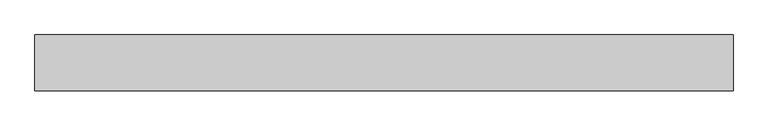
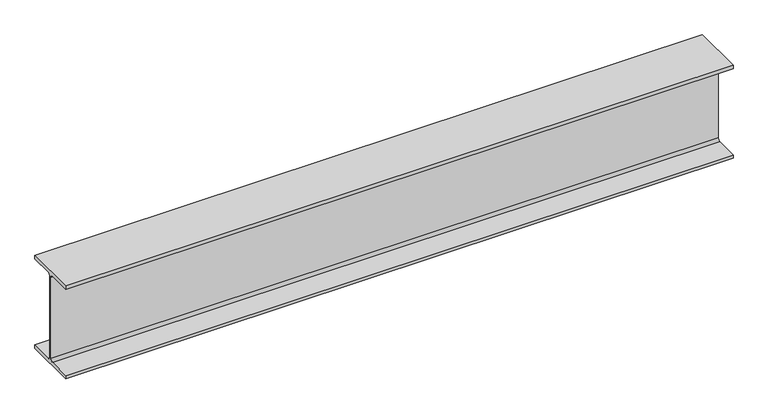
"""IFC4 building model written with IfcOpenShell, lengths in millimetres: beam geometry, Old_Steel Beam_H-KSD3502 : H_SB_ASB_H-194×150x6x9."""

from ifc_helpers import new_model, si_unit, point, frame, frame_2d, origin, place, context, project, spatial, polyline, circle_curve, trimmed, segment, composite_curve, outline, extrude, source, transform, mapped, element, save


def beam_5794e32c(model_context):
    return source(origin(), model_context, "Body", "SweptSolid", [
        extrude(outline(composite_curve([segment(polyline([(82.5, -141.5), (82.5, -151.7), (-82.5, -151.7), (-82.5, -141.5), (-11.9, -141.5)]), True, "CONTINUOUS"), segment(trimmed(circle_curve(frame_2d((-11.9, -132.6)), 8.9), [point((-11.9, -141.5))], [point((-3.0, -132.6))], True, "CARTESIAN"), True, "CONTINUOUS"), segment(polyline([(-3.0, -132.6), (-3.0, 132.6)]), True, "CONTINUOUS"), segment(trimmed(circle_curve(frame_2d((-11.9, 132.6)), 8.9), [point((-3.0, 132.6))], [point((-11.9, 141.5))], True, "CARTESIAN"), True, "CONTINUOUS"), segment(polyline([(-11.9, 141.5), (-82.5, 141.5), (-82.5, 151.7), (82.5, 151.7), (82.5, 141.5), (11.9, 141.5)]), True, "CONTINUOUS"), segment(trimmed(circle_curve(frame_2d((11.9, 132.6)), 8.9), [point((11.9, 141.5))], [point((3.0, 132.6))], True, "CARTESIAN"), True, "CONTINUOUS"), segment(polyline([(3.0, 132.6), (3.0, -132.6)]), True, "CONTINUOUS"), segment(trimmed(circle_curve(frame_2d((11.9, -132.6)), 8.9), [point((3.0, -132.6))], [point((11.9, -141.5))], True, "CARTESIAN"), True, "CONTINUOUS"), segment(polyline([(11.9, -141.5), (82.5, -141.5)]), True, "CONTINUOUS")], self_intersect=False)), frame((-1172.13, 0.0, 0.0), z_axis=(1.0, 0.0, 0.0), x_axis=(0.0, 1.0, 0.0)), (0.0, 0.0, 1.0), 2067.0467737),
    ])


if __name__ == "__main__":
    model = new_model("IFC4")
    model_context = context("Model", 3, world=origin())
    ifc_project = project(units=[si_unit("LENGTHUNIT", "METRE", prefix="MILLI")], contexts=[model_context])
    site = spatial("IfcSite", under=ifc_project)
    building = spatial("IfcBuilding", under=site)
    placement = place(None, origin())
    beam_shape = beam_5794e32c(model_context)
    element("IfcBeam", 1, ObjectType="Old_Steel Beam_H-KSD3502 : H_SB_ASB_H-194×150x6x9", at=placement, inside=building, context=model_context, shape_type="MappedRepresentation", body=[
        mapped(beam_shape, transform((0.0, 0.0, 0.0), x_axis=(1.0, 0.0, 0.0), y_axis=(0.0, 1.0, 0.0), z_axis=(0.0, 0.0, 1.0))),
    ])
    save(model, "model.ifc")

# Revit data of these elements
# Type "Old_Steel Beam_H-KSD3502 : H_SB_ASB_H-194×150x6x9"
#   Width = 15.0 cm
#   Web Thickness = 0.6 cm
#   Web Fillet = 1.3 cm
#   Warping Constant = 43316.0 cm⁶
#   Torsional Moment of Inertia = 8.622 cm⁴
#   Torsional Modulus = 1.0 cm³
#   Section Area = 39.01 cm²
#   Plastic Modulus weak axis = 104.0 cm³
#   Plastic Modulus strong axis = 309.0 cm³
#   Perimeter = 0.95 m²/m
#   Nominal Weight = 30.60 kgf/m
#   Moment of Inertia weak axis = 507.00 cm⁴
#   Moment of Inertia strong axis = 2690.00 cm⁴
#   Height = 19.4 cm
#   Flange Thickness = 0.9 cm
#   Elastic Modulus weak axis = 67.6 cm³
#   Elastic Modulus strong axis = 277.0 cm³
#   Centroid Vertical = 9.7 cm
#   Centroid Horizontal = 7.5 cm
#   Length [instance default] = 1.5240 m
#   Structural Material [instance default] = Steel, 45-345
#   Assembly Code = ""
# Element 1 (IfcBeam, "Old_Steel Beam_H-KSD3502 : H_SB_ASB_H-194×150x6x9")
#   Structural Material = none
# Materials
#   "Steel, 45-345": class "Metal", colour RGB 189 187 185, transparency 0, Description = "Steel 345 MPa", Cost = 0
